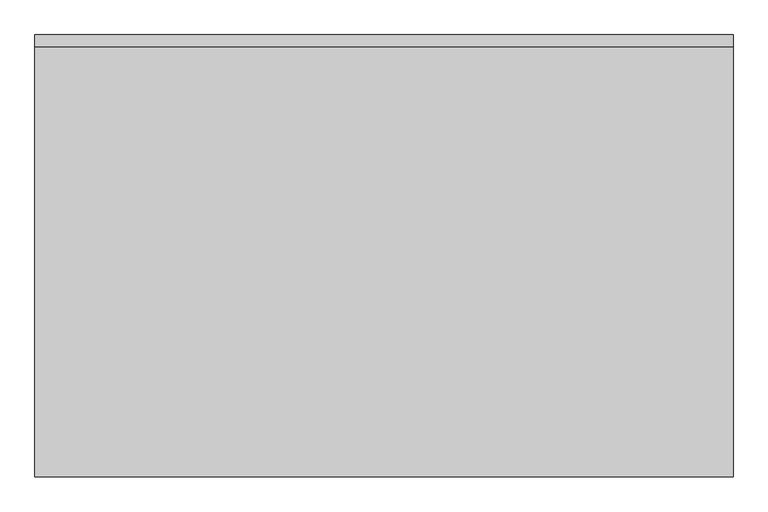
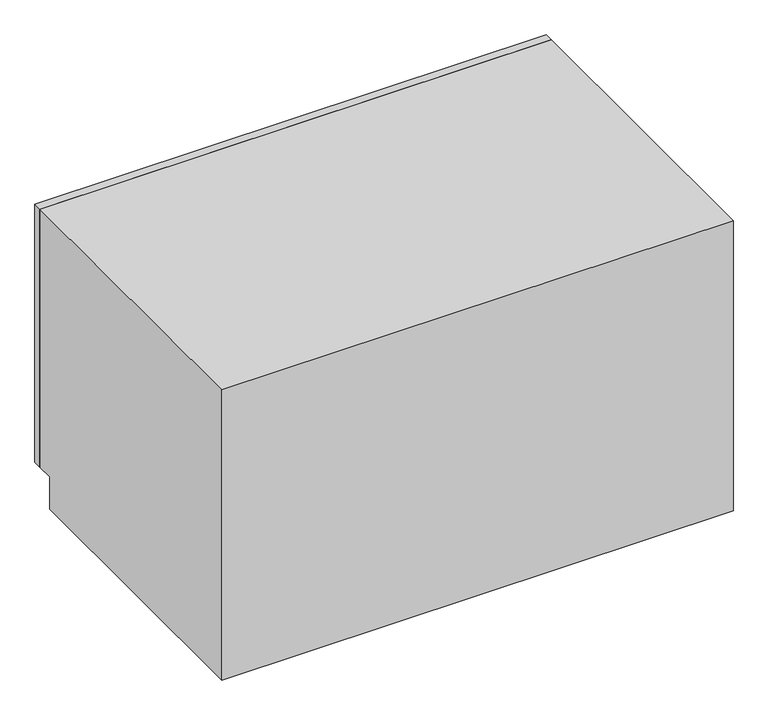
"""IFC4 building model written with IfcOpenShell, lengths in millimetres: furniture geometry, OD_CW_Base Cabinet : OD_CW_Base Cabinet."""

from ifc_helpers import new_model, si_unit, frame, origin, place, context, project, spatial, polyline, outline, extrude, source, transform, mapped, element, save


def furniture_14e7309d(model_context):
    return source(origin(), model_context, "Body", "SweptSolid", [
        extrude(outline(polyline([(18.7377049, 330.2), (18.7377049, 355.6), (1542.7377049, 355.6), (1542.7377049, 330.2), (18.7377049, 330.2)])), frame((0.0, 0.0, 101.6), z_axis=(0.0, 0.0, 1.0), x_axis=(1.0, 0.0, 0.0)), (0.0, 0.0, 1.0), 812.8),
        extrude(outline(polyline([(330.2, 914.4), (330.2, 101.6), (279.4, 101.6), (279.4, 0.0), (-609.6, 0.0), (-609.6, 914.4), (330.2, 914.4)])), frame((18.7377049, 0.0, 0.0), z_axis=(1.0, 0.0, 0.0), x_axis=(0.0, 1.0, 0.0)), (0.0, 0.0, 1.0), 1524.0),
    ])


if __name__ == "__main__":
    model = new_model("IFC4")
    model_context = context("Model", 3, world=origin())
    ifc_project = project(units=[si_unit("LENGTHUNIT", "METRE", prefix="MILLI")], contexts=[model_context])
    site = spatial("IfcSite", under=ifc_project)
    building = spatial("IfcBuilding", under=site)
    placement = place(None, origin())
    furniture_shape = furniture_14e7309d(model_context)
    element("IfcFurniture", 1, ObjectType="OD_CW_Base Cabinet : OD_CW_Base Cabinet", at=placement, inside=building, context=model_context, shape_type="MappedRepresentation", body=[
        mapped(furniture_shape, transform((0.0, 0.0, 0.0), x_axis=(1.0, 0.0, 0.0), y_axis=(0.0, 1.0, 0.0), z_axis=(0.0, 0.0, 1.0))),
    ])
    save(model, "model.ifc")

# Revit data of these elements
# Type "OD_CW_Base Cabinet : OD_CW_Base Cabinet"
#   OD_CW_Width [instance default] = 2' - 10"
#   OD_CW_Length [instance default] = 8' - 0"
#   OD_CW_Height [instance default] = 2' - 3"
#   Depth = 2' - 0"
#   Height = 3' - 0"
#   Width = 4' - 0"
#   OD_CW_Material_Front Panel [instance default] = none
#   OD_CW_Material_Body [instance default] = none
# Element 1 (IfcFurniture, "OD_CW_Base Cabinet : OD_CW_Base Cabinet")
#   OD_CW_Width = 3' - 2"
#   OD_CW_Length = 5' - 0"
#   OD_CW_Height = 3' - 0"
#   OD_CW_Material_Body = DISH SOIL TABLE
#   Materials on its faces: "DISH SOIL TABLE", "CASEWORK"
# Materials
#   "DISH SOIL TABLE": class "Generic", colour RGB 187 187 187, transparency 0, Cost = 0
#   "CASEWORK": class "Generic", colour RGB 181 181 181, transparency 0, Cost = 0
